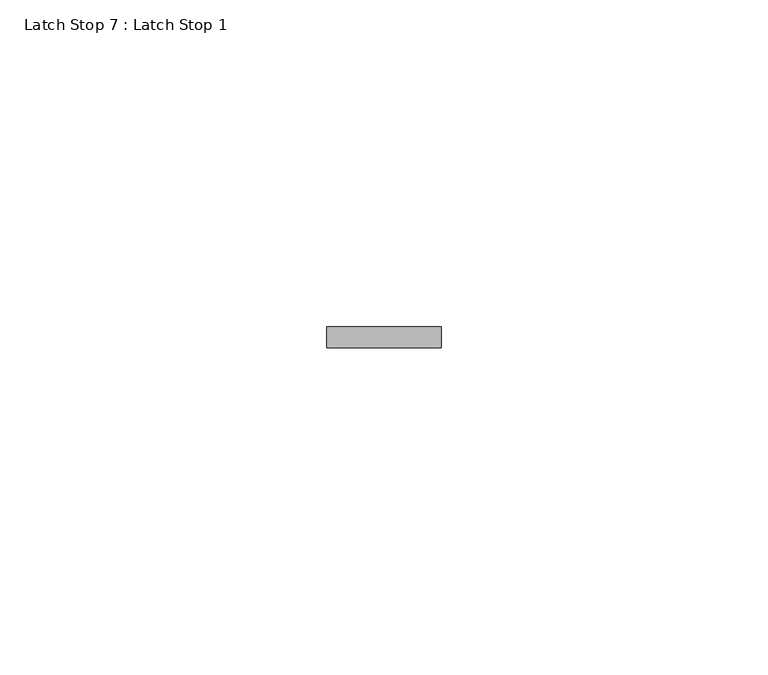
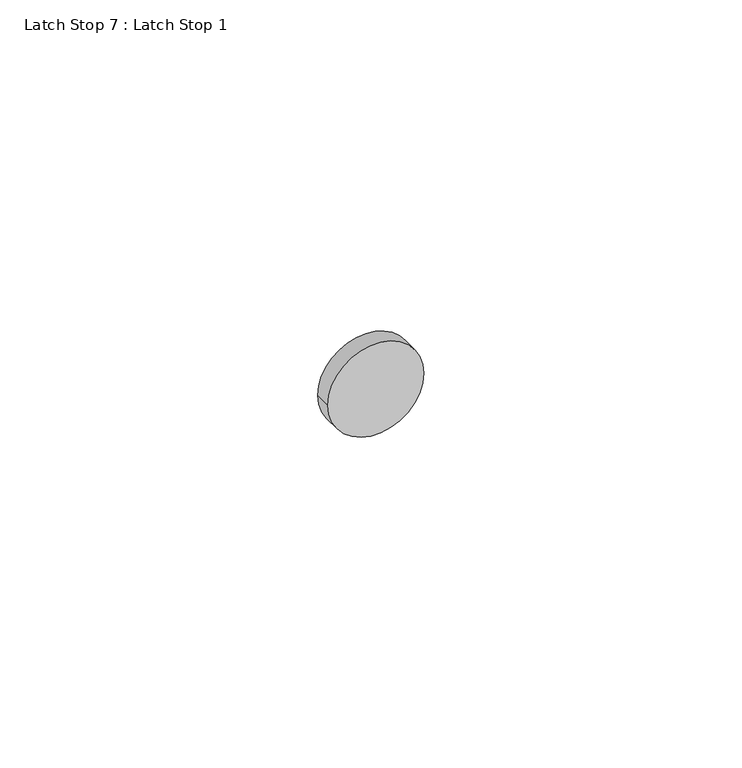
"""IFC4 building model written with IfcOpenShell, lengths in millimetres: proxy geometry, Latch Stop 7 : Latch Stop 1."""

from ifc_helpers import new_model, si_unit, point, frame, frame_2d, origin, place, context, project, spatial, circle_curve, trimmed, segment, composite_curve, outline, extrude, source, transform, mapped, element, save


def latch_stop_7_latch_stop_1_4e8d7d1d(model_context):
    return source(origin(), model_context, "Body", "SweptSolid", [
        extrude(outline(composite_curve([segment(trimmed(circle_curve(frame_2d((1066.8, 587312.7185739)), 8.73125), [point((1066.8, 587303.9873239))], [point((1066.8, 587321.4498239))], False, "CARTESIAN"), True, "CONTINUOUS"), segment(trimmed(circle_curve(frame_2d((1066.8, 587312.7185739)), 8.73125), [point((1066.8, 587321.4498239))], [point((1066.8, 587303.9873239))], False, "CARTESIAN"), True, "CONTINUOUS")], self_intersect=False)), frame((0.0, -535166.6413841, 0.0), z_axis=(0.0, 1.0, 0.0), x_axis=(0.0, 0.0, 1.0)), (0.0, 0.0, 1.0), 3.175),
    ])


if __name__ == "__main__":
    model = new_model("IFC4")
    model_context = context("Model", 3, world=origin())
    ifc_project = project(units=[si_unit("LENGTHUNIT", "METRE", prefix="MILLI")], contexts=[model_context])
    site = spatial("IfcSite", under=ifc_project)
    building = spatial("IfcBuilding", under=site)
    placement = place(None, origin())
    latch_stop_7_latch_stop_1_shape = latch_stop_7_latch_stop_1_4e8d7d1d(model_context)
    element("IfcBuildingElementProxy", 1, Name="Latch Stop 7 : Latch Stop 1", ObjectType="Latch Stop 7 : Latch Stop 1", at=placement, inside=building, context=model_context, shape_type="MappedRepresentation", body=[
        mapped(latch_stop_7_latch_stop_1_shape, transform((0.0, 0.0, 0.0), x_axis=(1.0, 0.0, 0.0), y_axis=(0.0, 1.0, 0.0), z_axis=(0.0, 0.0, 1.0))),
    ])
    save(model, "model.ifc")

# Revit data of these elements
# Element 1 (IfcBuildingElementProxy, "Latch Stop 7 : Latch Stop 1")
#   Materials on its faces: "GALV. GATE LATCH"
# Materials
#   "GALV. GATE LATCH": class "Metal", colour RGB 189 187 185, transparency 0, Description = "Carbon steel", Cost = 0
